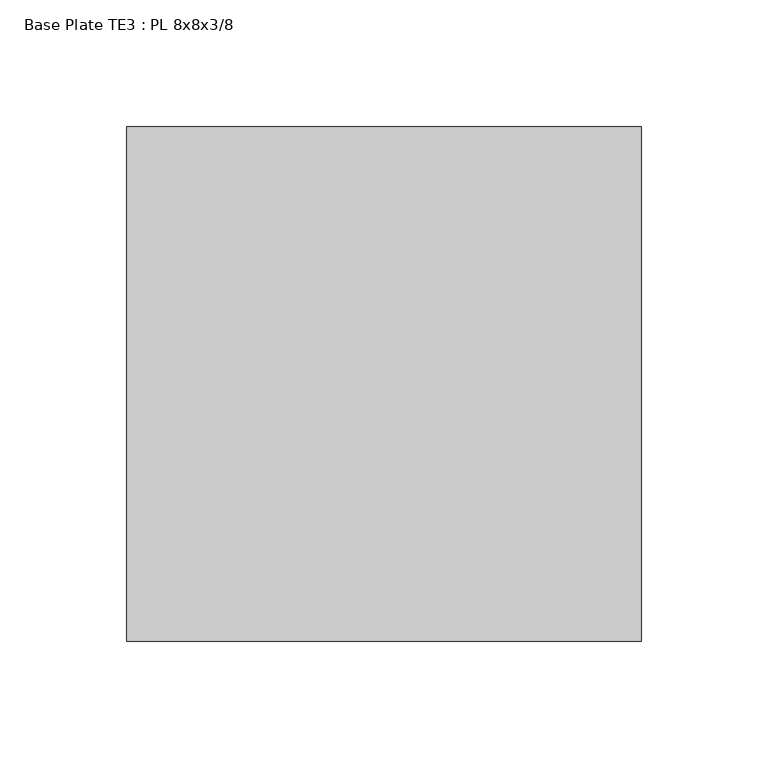
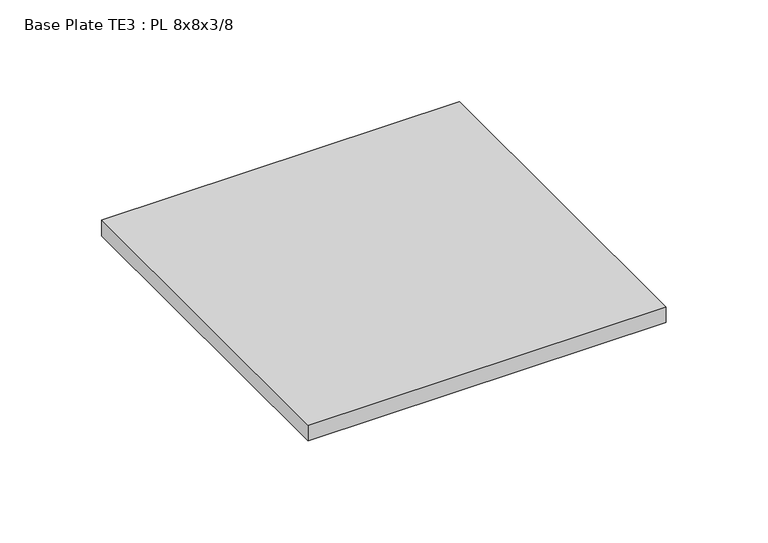
"""IFC4 building model written with IfcOpenShell, lengths in millimetres: proxy geometry, Base Plate TE3 : PL 8x8x3/8."""

from ifc_helpers import new_model, si_unit, frame, origin, place, context, project, spatial, polyline, outline, extrude, source, transform, mapped, element, save


def base_plate_te3_pl_8x8x3_8_af136eb6(model_context):
    return source(origin(), model_context, "Body", "SweptSolid", [
        extrude(outline(polyline([(590318.6599233, -535103.1413841), (590318.6599233, -535306.3413841), (590115.4599233, -535306.3413841), (590115.4599233, -535103.1413841), (590318.6599233, -535103.1413841)])), frame((0.0, 0.0, 19.05), z_axis=(0.0, 0.0, 1.0), x_axis=(1.0, 0.0, 0.0)), (0.0, 0.0, 1.0), 9.525),
    ])


if __name__ == "__main__":
    model = new_model("IFC4")
    model_context = context("Model", 3, world=origin())
    ifc_project = project(units=[si_unit("LENGTHUNIT", "METRE", prefix="MILLI")], contexts=[model_context])
    site = spatial("IfcSite", under=ifc_project)
    building = spatial("IfcBuilding", under=site)
    placement = place(None, origin())
    base_plate_te3_pl_8x8x3_8_shape = base_plate_te3_pl_8x8x3_8_af136eb6(model_context)
    element("IfcBuildingElementProxy", 1, Name="Base Plate TE3 : PL 8x8x3/8", ObjectType="Base Plate TE3 : PL 8x8x3/8", at=placement, inside=building, context=model_context, shape_type="MappedRepresentation", body=[
        mapped(base_plate_te3_pl_8x8x3_8_shape, transform((0.0, 0.0, 0.0), x_axis=(1.0, 0.0, 0.0), y_axis=(0.0, 1.0, 0.0), z_axis=(0.0, 0.0, 1.0))),
    ])
    save(model, "model.ifc")

# Revit data of these elements
# Element 1 (IfcBuildingElementProxy, "Base Plate TE3 : PL 8x8x3/8")
#   Materials on its faces: "GALV. STL BASE PLATE"
# Materials
#   "GALV. STL BASE PLATE": class "Generic", colour RGB 211 211 207, transparency 0, Cost = 0
